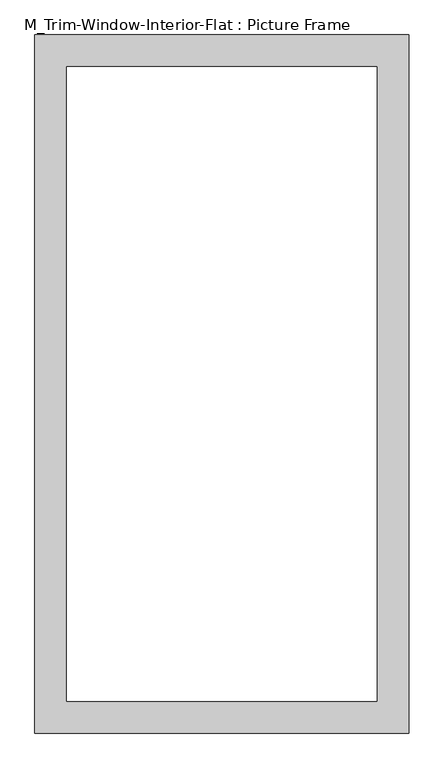
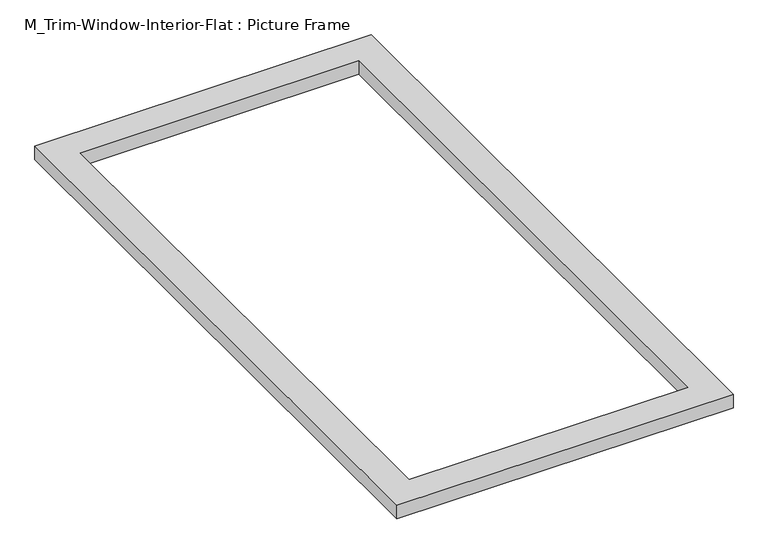
"""IFC4 building model written with IfcOpenShell, lengths in millimetres: proxy geometry, M_Trim-Window-Interior-Flat : Picture Frame."""

from ifc_helpers import new_model, si_unit, origin, origin_with_axes, place, context, project, spatial, polyline, outline, extrude, source, transform, mapped, element, save


def m_trim_window_interior_flat_picture_frame_289146a9(model_context):
    return source(origin(), model_context, "Body", "SweptSolid", [
        extrude(outline(polyline([(352.1, 47.3), (352.1, -1266.5), (-352.1, -1266.5), (-352.1, 47.3), (352.1, 47.3)]), holes=[polyline([(292.1, -12.7), (-292.1, -12.7), (-292.1, -1206.5), (292.1, -1206.5), (292.1, -12.7)])]), origin_with_axes(), (0.0, 0.0, 1.0), 30.0),
    ])


if __name__ == "__main__":
    model = new_model("IFC4")
    model_context = context("Model", 3, world=origin())
    ifc_project = project(units=[si_unit("LENGTHUNIT", "METRE", prefix="MILLI")], contexts=[model_context])
    site = spatial("IfcSite", under=ifc_project)
    building = spatial("IfcBuilding", under=site)
    placement = place(None, origin())
    m_trim_window_interior_flat_picture_frame_shape = m_trim_window_interior_flat_picture_frame_289146a9(model_context)
    element("IfcBuildingElementProxy", 1, Name="M_Trim-Window-Interior-Flat : Picture Frame", ObjectType="M_Trim-Window-Interior-Flat : Picture Frame", at=placement, inside=building, context=model_context, shape_type="MappedRepresentation", body=[
        mapped(m_trim_window_interior_flat_picture_frame_shape, transform((0.0, 0.0, 0.0), x_axis=(1.0, 0.0, 0.0), y_axis=(0.0, 1.0, 0.0), z_axis=(0.0, 0.0, 1.0))),
    ])
    save(model, "model.ifc")

# Revit data of these elements
# Type "M_Trim-Window-Interior-Flat : Picture Frame"
#   Trim Thickness_Picture Frame = 0' - 1.1811"
#   Trim Width = 0' - 2.3622"
#   Trim Thickness_with Sill = 0' - 0.7874"
#   Sill Thickness = 0' - 1.1811"
#   Opening Width [instance default] = 1' - 11.62205"
#   Opening Height [instance default] = 2' - 11.43307"
#   Default Elevation = 3' - 11.24409"
#   Sill = no
#   Picture Frame = yes
#   Trim Material [instance default] = none
# Element 1 (IfcBuildingElementProxy, "M_Trim-Window-Interior-Flat : Picture Frame")
#   Opening Width = 2' - 0"
#   Opening Height = 4' - 0"
#   Trim Material = Wood - Stained
#   Materials on its faces: "Wood - Stained"
# Materials
#   "Wood - Stained": class "Wood", colour RGB 224 178 126, transparency 0, Cost = 0
